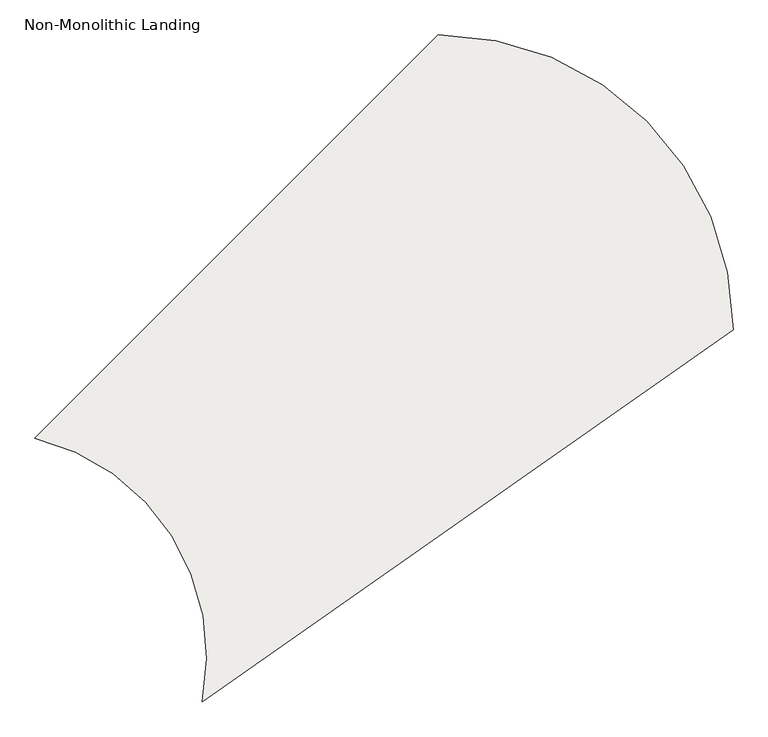
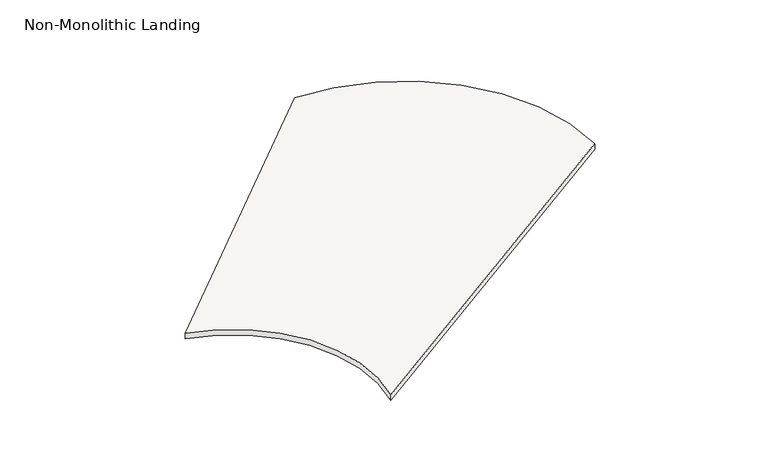
"""IFC4 building model written with IfcOpenShell, lengths in millimetres: slab geometry, Non-Monolithic Landing."""

from ifc_helpers import new_model, si_unit, point, frame, frame_2d, origin, place, context, project, spatial, polyline, circle_curve, trimmed, segment, composite_curve, outline, extrude, source, transform, mapped, element, save


def non_monolithic_landing_42941364(model_context):
    return source(origin(), model_context, "Body", "SweptSolid", [
        extrude(outline(composite_curve([segment(polyline([(20712.2483022, 45217.3358181), (22937.9067224, 47442.9942383)]), True, "CONTINUOUS"), segment(trimmed(circle_curve(frame_2d((22937.9067224, 45816.6486415)), 1626.3455967), [point((22937.9067224, 47442.9942383))], [point((24564.2523191, 45816.6486415))], False, "CARTESIAN"), True, "CONTINUOUS"), segment(polyline([(24564.2523191, 45816.6486415), (21634.7503997, 43763.8153492)]), True, "CONTINUOUS"), segment(trimmed(circle_curve(frame_2d((20426.3929767, 44016.4115026)), 1234.476601), [point((21634.7503997, 43763.8153492))], [point((20712.2483022, 45217.3358181))], True, "CARTESIAN"), True, "CONTINUOUS")], self_intersect=False)), frame((0.0, 0.0, 12880.2325581), z_axis=(0.0, 0.0, 1.0), x_axis=(1.0, 0.0, 0.0)), (0.0, 0.0, 1.0), 50.0),
    ])


if __name__ == "__main__":
    model = new_model("IFC4")
    model_context = context("Model", 3, world=origin())
    ifc_project = project(units=[si_unit("LENGTHUNIT", "METRE", prefix="MILLI")], contexts=[model_context])
    site = spatial("IfcSite", under=ifc_project)
    building = spatial("IfcBuilding", under=site)
    placement = place(None, origin())
    non_monolithic_landing_shape = non_monolithic_landing_42941364(model_context)
    element("IfcSlab", 1, ObjectType="Non-Monolithic Landing", at=placement, inside=building, context=model_context, shape_type="MappedRepresentation", body=[
        mapped(non_monolithic_landing_shape, transform((0.0, 0.0, 0.0), x_axis=(1.0, 0.0, 0.0), y_axis=(0.0, 1.0, 0.0), z_axis=(0.0, 0.0, 1.0))),
    ])
    save(model, "model.ifc")

# Revit data of these elements
# Project information
#   Project Issue Date = "Issue Date"
#   Project Status = "Project Status"
#   Client Name = "Owner"
#   Project Address = "Enter address here"
#   Project Name = "Project Name"
#   Project Number = "0001"
